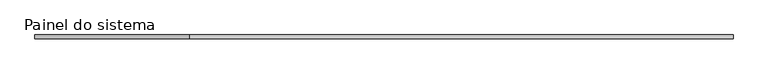
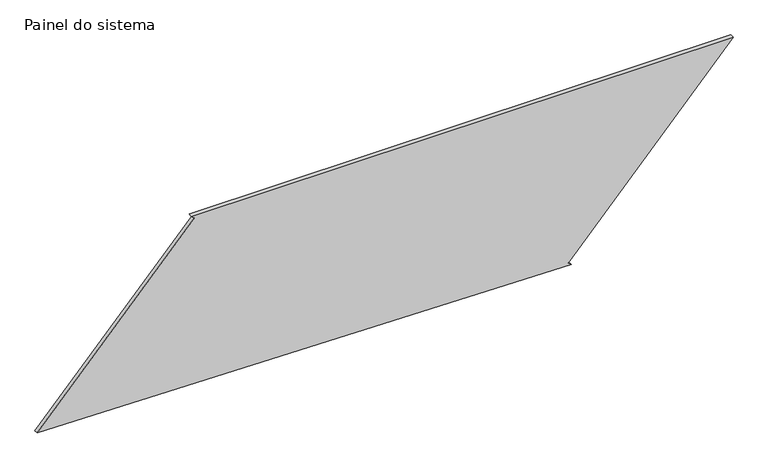
"""IFC4 building model written with IfcOpenShell, lengths in millimetres: plate geometry, Painel do sistema : Envidraçado."""

from ifc_helpers import new_model, si_unit, frame, origin, place, context, project, spatial, polyline, outline, extrude, source, transform, mapped, element, save


def painel_do_sistema_dfe40748(model_context):
    return source(origin(), model_context, "Body", "SweptSolid", [
        extrude(outline(polyline([(0.0, 1182.9203685), (16.8339598, 1164.4374629), (1168.5868451, 2213.4371321), (1168.5868451, -1232.4887988), (1151.7528853, -1214.0058933), (54.4238329, -2213.4371321), (0.0, 1182.9203685)])), frame((0.0, 24.5, 0.0), z_axis=(0.0, 1.0, 0.0), x_axis=(0.0, 0.0, 1.0)), (0.0, 0.0, 1.0), 25.0),
    ])


if __name__ == "__main__":
    model = new_model("IFC4")
    model_context = context("Model", 3, world=origin())
    ifc_project = project(units=[si_unit("LENGTHUNIT", "METRE", prefix="MILLI")], contexts=[model_context])
    site = spatial("IfcSite", under=ifc_project)
    building = spatial("IfcBuilding", under=site)
    placement = place(None, origin())
    painel_do_sistema_shape = painel_do_sistema_dfe40748(model_context)
    element("IfcPlate", 1, ObjectType="Painel do sistema : Envidraçado", at=placement, inside=building, context=model_context, shape_type="MappedRepresentation", body=[
        mapped(painel_do_sistema_shape, transform((0.0, 0.0, 0.0), x_axis=(1.0, 0.0, 0.0), y_axis=(0.0, 1.0, 0.0), z_axis=(0.0, 0.0, 1.0))),
    ])
    save(model, "model.ifc")

# Revit data of these elements
# Type "Painel do sistema : Envidraçado"
#   Construction Type Id = "GSP4R"
#   Analytic Construction = "Vidraça única Pilkington 1/8 pol"
#   Visual Light Transmittance = 0.9
#   Solar Heat Gain Coefficient = 0.86
#   Heat Transfer Coefficient (U) = 6.7069 W/(m²·K)
# Element 1 (IfcPlate, "Painel do sistema : Envidraçado")
#   Materials on its faces: "Vidro"
# Materials
#   "Vidro": class "Vidro", colour RGB 0 128 192, transparency 0.9, Description = "Vidro de sílica", Cost = 0
